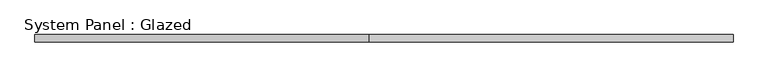
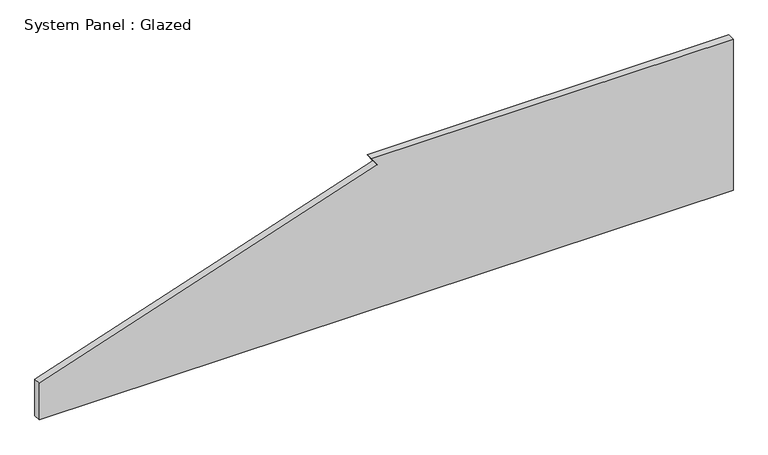
"""IFC4 building model written with IfcOpenShell, lengths in millimetres: plate geometry, System Panel : Glazed."""

from ifc_helpers import new_model, si_unit, frame, origin, place, context, project, spatial, polyline, outline, extrude, source, transform, mapped, element, save


def system_panel_glazed_5992a3c5(model_context):
    return source(origin(), model_context, "Body", "SweptSolid", [
        extrude(outline(polyline([(0.0, -1187.45), (0.0, 1187.45), (546.1, 1187.45), (546.1, -50.8), (517.6086106, -30.7195369), (132.0317895, -1187.45), (0.0, -1187.45)])), frame((0.0, -44.45, 0.0), z_axis=(0.0, 1.0, 0.0), x_axis=(0.0, 0.0, 1.0)), (0.0, 0.0, 1.0), 25.4),
    ])


if __name__ == "__main__":
    model = new_model("IFC4")
    model_context = context("Model", 3, world=origin())
    ifc_project = project(units=[si_unit("LENGTHUNIT", "METRE", prefix="MILLI")], contexts=[model_context])
    site = spatial("IfcSite", under=ifc_project)
    building = spatial("IfcBuilding", under=site)
    placement = place(None, origin())
    system_panel_glazed_shape = system_panel_glazed_5992a3c5(model_context)
    element("IfcPlate", 1, ObjectType="System Panel : Glazed", at=placement, inside=building, context=model_context, shape_type="MappedRepresentation", body=[
        mapped(system_panel_glazed_shape, transform((0.0, 0.0, 0.0), x_axis=(1.0, 0.0, 0.0), y_axis=(0.0, 1.0, 0.0), z_axis=(0.0, 0.0, 1.0))),
    ])
    save(model, "model.ifc")

# Revit data of these elements
# Element 1 (IfcPlate, "System Panel : Glazed")
#   Materials on its faces: "Glass"
# Materials
#   "Glass": class "Glass", colour RGB 0 128 192, transparency 0.75
